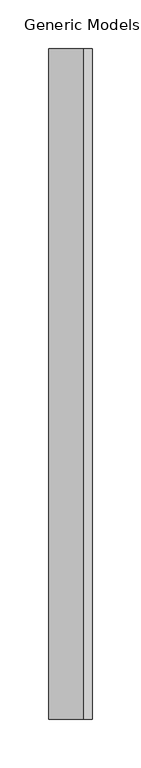
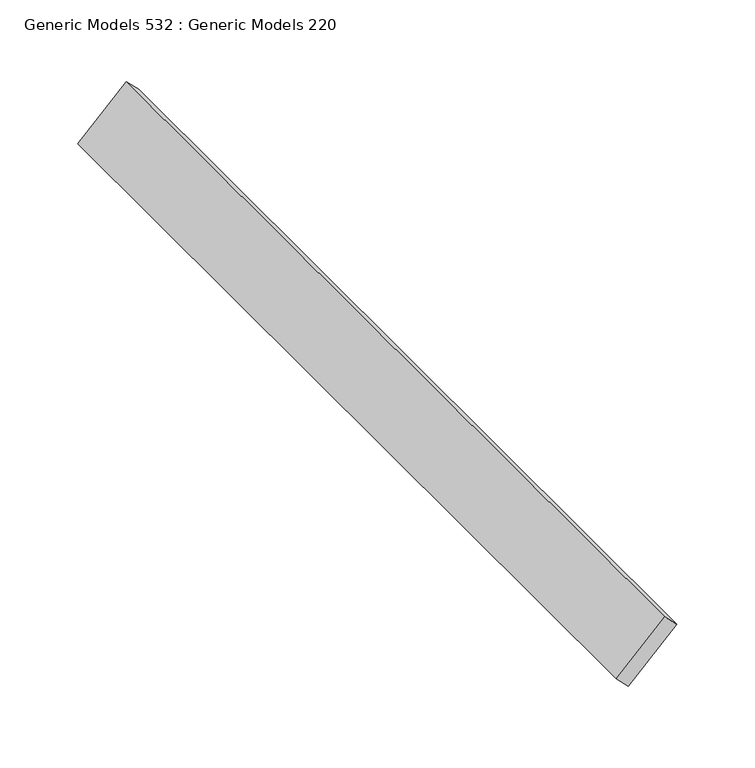
"""IFC4 building model written with IfcOpenShell, lengths in millimetres: proxy geometry, Generic Models 532 : Generic Models 220."""

from ifc_helpers import new_model, si_unit, frame, origin, place, context, project, spatial, polyline, outline, extrude, source, transform, mapped, element, save


def generic_models_532_generic_models_220_c9ed0bd9(model_context):
    return source(origin(), model_context, "Body", "SweptSolid", [
        extrude(outline(polyline([(0.0, -12.7000001), (0.0, 0.0), (690.8142348, 0.0), (690.8142348, -12.7000001), (0.0, -12.7000001)])), frame((7841.3059863, 4539.4872686, 125255.6399101), z_axis=(0.7071067811868034, 0.0, 0.7071067811862918), x_axis=(0.0, -1.0, 0.0)), (0.0, 0.0, 1.0), 50.8),
    ])


if __name__ == "__main__":
    model = new_model("IFC4")
    model_context = context("Model", 3, world=origin())
    ifc_project = project(units=[si_unit("LENGTHUNIT", "METRE", prefix="MILLI")], contexts=[model_context])
    site = spatial("IfcSite", under=ifc_project)
    building = spatial("IfcBuilding", under=site)
    placement = place(None, origin())
    generic_models_532_generic_models_220_shape = generic_models_532_generic_models_220_c9ed0bd9(model_context)
    element("IfcBuildingElementProxy", 1, Name="Generic Models 532 : Generic Models 220", ObjectType="Generic Models 532 : Generic Models 220", at=placement, inside=building, context=model_context, shape_type="MappedRepresentation", body=[
        mapped(generic_models_532_generic_models_220_shape, transform((0.0, 0.0, 0.0), x_axis=(1.0, 0.0, 0.0), y_axis=(0.0, 1.0, 0.0), z_axis=(0.0, 0.0, 1.0))),
    ])
    save(model, "model.ifc")

# Revit data of these elements
# Element 1 (IfcBuildingElementProxy, "Generic Models 532 : Generic Models 220")
#   Materials on its faces: "_WOOD TONE ALUMINUM EXTRUSION SLAT BY KNOTWOOD"
# Materials
#   "_WOOD TONE ALUMINUM EXTRUSION SLAT BY KNOTWOOD": class "Generic", colour RGB 177 130 114, transparency 0, Cost = 0
